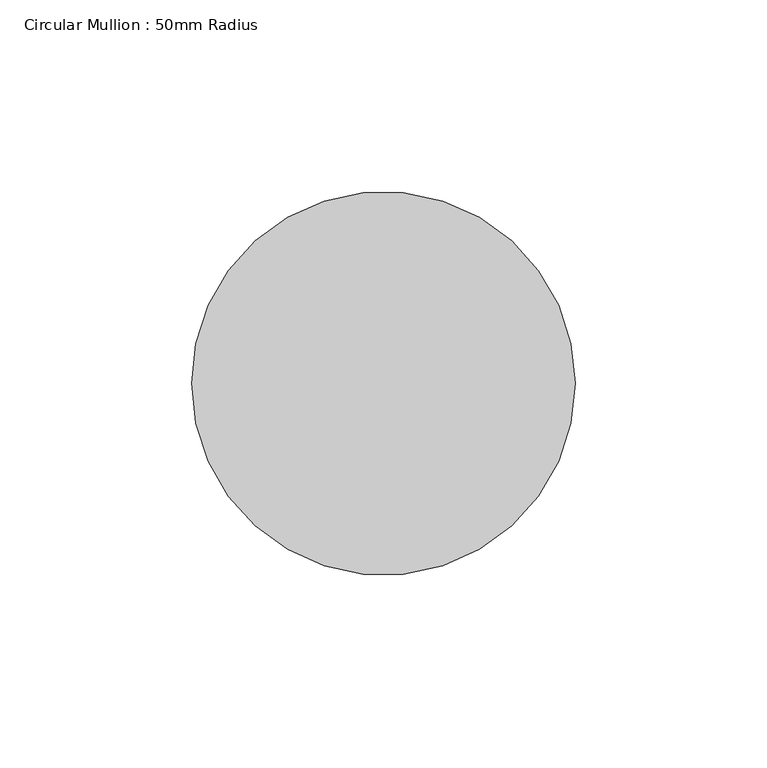
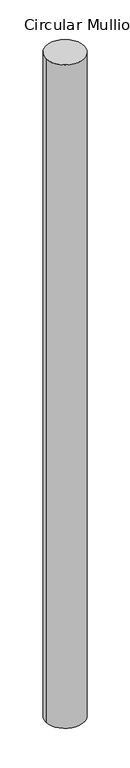
"""IFC4 building model written with IfcOpenShell, lengths in millimetres: member geometry, Circular Mullion : 50mm Radius."""

from ifc_helpers import new_model, si_unit, point, frame, origin, origin_2d, place, context, project, spatial, circle_curve, trimmed, segment, composite_curve, outline, extrude, source, transform, mapped, element, save


def circular_mullion_50mm_radius_9b437c65(model_context):
    return source(origin(), model_context, "Body", "SweptSolid", [
        extrude(outline(composite_curve([segment(trimmed(circle_curve(origin_2d(), 50.0), [point((50.0, 0.0))], [point((-50.0, 0.0))], False, "CARTESIAN"), True, "CONTINUOUS"), segment(trimmed(circle_curve(origin_2d(), 50.0), [point((-50.0, 0.0))], [point((50.0, 0.0))], False, "CARTESIAN"), True, "CONTINUOUS")], self_intersect=False)), frame((0.0, 0.0, -1825.2603389), z_axis=(0.0, 0.0, 1.0), x_axis=(1.0, 0.0, 0.0)), (0.0, 0.0, 1.0), 1825.2603389),
    ])


if __name__ == "__main__":
    model = new_model("IFC4")
    model_context = context("Model", 3, world=origin())
    ifc_project = project(units=[si_unit("LENGTHUNIT", "METRE", prefix="MILLI")], contexts=[model_context])
    site = spatial("IfcSite", under=ifc_project)
    building = spatial("IfcBuilding", under=site)
    placement = place(None, origin())
    circular_mullion_50mm_radius_shape = circular_mullion_50mm_radius_9b437c65(model_context)
    element("IfcMember", 1, ObjectType="Circular Mullion : 50mm Radius", at=placement, inside=building, context=model_context, shape_type="MappedRepresentation", body=[
        mapped(circular_mullion_50mm_radius_shape, transform((0.0, 0.0, 0.0), x_axis=(1.0, 0.0, 0.0), y_axis=(0.0, 1.0, 0.0), z_axis=(0.0, 0.0, 1.0))),
    ])
    save(model, "model.ifc")

# Revit data of these elements
# Type "Circular Mullion : 50mm Radius"
#   built-in parameter 1007350 = 0.164042 (stored number, unit not read)
# Element 1 (IfcMember, "Circular Mullion : 50mm Radius")
#   Materials on its faces: "Aluminium"
# Materials
#   "Aluminium": class "Metal", colour RGB 247 247 247, transparency 0, Description = "Aluminium 6061", Cost = 0
